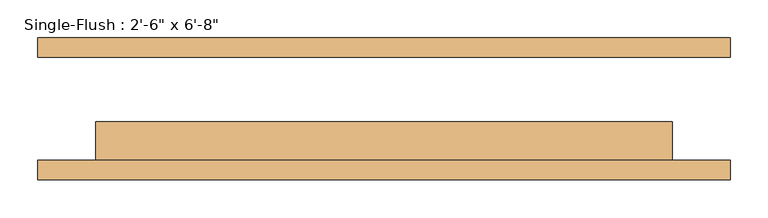
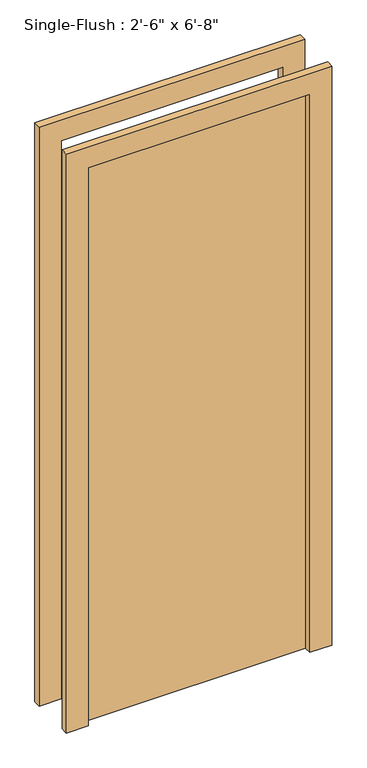
"""IFC4 building model written with IfcOpenShell, lengths in millimetres: door geometry."""

import ifcopenshell
import ifcopenshell.guid

model = None  # the IFC model being written
_history = None  # IfcOwnerHistory: only IFC2X3 demands one
_inside = {}  # id of a spatial element -> (the spatial element, [elements in it])
_under = {}  # id of a project, library or spatial element -> (it, [spatial elements below it])
_declared = {}  # id of a project -> (the project, [libraries it declares])
_typed = {}  # id of a type object -> (the type object, [elements of that type])
_made_of = {}  # id of a material, layer set ... -> (it, [elements and type objects made of it])


def new_model(schema):
    """Start an empty IFC model of exactly this schema.

    Asked for "IFC4X3", IfcOpenShell would pick the latest addendum, in which some entities
    have other attributes; the version numbers below select the first issue.
    IFC2X3 requires an IfcOwnerHistory on every rooted entity: one is made here for all.
    """
    global model, _history
    if schema == "IFC4X3":
        model = ifcopenshell.file(schema_version=(4, 3, 0, 0))
    else:
        model = ifcopenshell.file(schema=schema)
    _inside.clear()
    _under.clear()
    _declared.clear()
    _typed.clear()
    _made_of.clear()
    _history = None
    if model.schema == "IFC2X3":
        org = make("IfcOrganization", Name="unknown")
        user = make(
            "IfcPersonAndOrganization",
            ThePerson=make("IfcPerson", FamilyName="unknown"),
            TheOrganization=org,
        )
        app = make(
            "IfcApplication",
            ApplicationDeveloper=org,
            Version="unknown",
            ApplicationFullName="unknown",
            ApplicationIdentifier="unknown",
        )
        _history = make(
            "IfcOwnerHistory",
            OwningUser=user,
            OwningApplication=app,
            ChangeAction="ADDED",
            CreationDate=0,
        )
    return model


def make(cls, **values):
    """One entity of the class cls with the attributes given. An attribute that is None is left unset."""
    return model.create_entity(
        cls, **{name: value for name, value in values.items() if value is not None}
    )


def rooted(cls, **values):
    """An entity with a GlobalId (a new one), such as an element, a storey or a relation."""
    return make(cls, GlobalId=ifcopenshell.guid.new(), OwnerHistory=_history, **values)


def si_unit(unit_type, name, prefix=None):
    """IfcSIUnit, for example si_unit("LENGTHUNIT", "METRE", prefix="MILLI")."""
    return make("IfcSIUnit", UnitType=unit_type, Prefix=prefix, Name=name)


def assignment(units):
    """IfcUnitAssignment: the units of a project."""
    return None if units is None else make("IfcUnitAssignment", Units=units)


def point(xyz):
    """IfcCartesianPoint."""
    return None if xyz is None else make("IfcCartesianPoint", Coordinates=xyz)


def direction(xyz):
    """IfcDirection."""
    return None if xyz is None else make("IfcDirection", DirectionRatios=xyz)


def frame(location, z_axis=None, x_axis=None):
    """IfcAxis2Placement3D, a coordinate frame: its origin and axes. An axis left out is left unset."""
    return make(
        "IfcAxis2Placement3D",
        Location=point(location),
        Axis=direction(z_axis),
        RefDirection=direction(x_axis),
    )


def origin():
    """The frame at (0, 0, 0) with its axes left unset."""
    return frame((0.0, 0.0, 0.0))


def origin_with_axes():
    """The frame at (0, 0, 0) with the z axis (0, 0, 1) and the x axis (1, 0, 0) written out."""
    return frame((0.0, 0.0, 0.0), z_axis=(0.0, 0.0, 1.0), x_axis=(1.0, 0.0, 0.0))


def place(relative_to, where):
    """IfcLocalPlacement: puts the frame where relative to a parent placement (None: the world)."""
    return make(
        "IfcLocalPlacement", PlacementRelTo=relative_to, RelativePlacement=where
    )


def context(
    kind, dimensions, precision=None, world=None, true_north=None, identifier=None
):
    """IfcGeometricRepresentationContext, for example the 3D "Model" context."""
    return make(
        "IfcGeometricRepresentationContext",
        ContextIdentifier=identifier,
        ContextType=kind,
        CoordinateSpaceDimension=dimensions,
        Precision=precision,
        WorldCoordinateSystem=world,
        TrueNorth=true_north,
    )


def project(units=None, contexts=None):
    """IfcProject with its units and contexts."""
    return rooted(
        "IfcProject",
        Name="project",
        RepresentationContexts=contexts,
        UnitsInContext=assignment(units),
    )


def spatial(cls, under=None, at=None, **own):
    """A site, building, storey or space (cls), placed at a placement, below another one or the project."""
    s = rooted(cls, ObjectPlacement=at, **own)
    if under is not None:
        _under.setdefault(under.id(), (under, []))[1].append(s)
    return s


def polyline(points):
    """IfcPolyline through the points."""
    return make("IfcPolyline", Points=[point(p) for p in points])


def outline(outer, holes=None, kind="AREA"):
    """IfcArbitraryClosedProfileDef: a profile drawn as a closed curve; with holes, ...WithVoids."""
    if holes is None:
        return make("IfcArbitraryClosedProfileDef", ProfileType=kind, OuterCurve=outer)
    return make(
        "IfcArbitraryProfileDefWithVoids",
        ProfileType=kind,
        OuterCurve=outer,
        InnerCurves=holes,
    )


def extrude(swept, where, along, depth):
    """IfcExtrudedAreaSolid: the profile swept, set in the frame where, extruded along a direction by depth."""
    return make(
        "IfcExtrudedAreaSolid",
        SweptArea=swept,
        Position=where,
        ExtrudedDirection=direction(along),
        Depth=depth,
    )


def shape(context_of_items, identifier, shape_type, items):
    """IfcShapeRepresentation: the items that make up one representation, for example the "Body"."""
    return make(
        "IfcShapeRepresentation",
        ContextOfItems=context_of_items,
        RepresentationIdentifier=identifier,
        RepresentationType=shape_type,
        Items=items,
    )


def source(mapping_origin, context_of_items, identifier, shape_type, items):
    """IfcRepresentationMap: a shape defined once, which mapped items show again and again."""
    return make(
        "IfcRepresentationMap",
        MappingOrigin=mapping_origin,
        MappedRepresentation=shape(context_of_items, identifier, shape_type, items),
    )


def transform(
    local_origin,
    x_axis=None,
    y_axis=None,
    z_axis=None,
    scale=None,
    scale2=None,
    scale3=None,
    uniform=True,
):
    """IfcCartesianTransformationOperator3D, or its non-uniform kind. x_axis, y_axis, z_axis: its Axis1, 2, 3."""
    if uniform:
        return make(
            "IfcCartesianTransformationOperator3D",
            Axis1=direction(x_axis),
            Axis2=direction(y_axis),
            LocalOrigin=point(local_origin),
            Scale=scale,
            Axis3=direction(z_axis),
        )
    return make(
        "IfcCartesianTransformationOperator3DnonUniform",
        Axis1=direction(x_axis),
        Axis2=direction(y_axis),
        LocalOrigin=point(local_origin),
        Scale=scale,
        Axis3=direction(z_axis),
        Scale2=scale2,
        Scale3=scale3,
    )


def mapped(mapping_source, mapping_target):
    """IfcMappedItem: shows the shape of a source again, moved by a transform."""
    return make(
        "IfcMappedItem", MappingSource=mapping_source, MappingTarget=mapping_target
    )


def made_of(thing, what):
    """Note that an element or type object is made of a material, layer set ...; save() writes the relation."""
    if what is not None:
        _made_of.setdefault(what.id(), (what, []))[1].append(thing)
    return thing


def element(
    cls,
    number,
    at=None,
    inside=None,
    cuts=None,
    type_object=None,
    material=None,
    context=None,
    identifier="Body",
    shape_type=None,
    held_by="IfcProductDefinitionShape",
    body=None,
    shapes=None,
    **own,
):
    """One element of the class cls, such as IfcWall. Its Tag is "e" and its number.

    at: its placement. inside: the storey or other place that contains it. cuts: it is an
    opening in that element (IfcRelVoidsElement). A single representation is given by context,
    identifier, shape_type and body (its items); several are given by shapes. held_by: the class
    of the entity that holds the representations. save() writes the other relations.
    """
    e = rooted(cls, Tag="e%d" % number, ObjectPlacement=at, **own)
    if body is not None:
        shapes = [shape(context, identifier, shape_type, body)]
    if shapes is not None:
        e.Representation = make(held_by, Representations=shapes)
    if inside is not None:
        _inside.setdefault(inside.id(), (inside, []))[1].append(e)
    if cuts is not None:
        rooted(
            "IfcRelVoidsElement", RelatingBuildingElement=cuts, RelatedOpeningElement=e
        )
    if type_object is not None:
        _typed.setdefault(type_object.id(), (type_object, []))[1].append(e)
    return made_of(e, material)


def aggregate(whole, parts):
    """IfcRelAggregates: a whole, such as a stair, and the parts it consists of."""
    return rooted("IfcRelAggregates", RelatingObject=whole, RelatedObjects=parts)


def save(model, path):
    """Write the relations noted so far, then the file.

    IfcRelAggregates (storeys below a building ...), IfcRelContainedInSpatialStructure (elements
    in a storey), IfcRelDefinesByType, IfcRelAssociatesMaterial and IfcRelDeclares: one each for
    every whole, place, type object, material and project.
    """
    for whole, parts in _under.values():
        aggregate(whole, parts)
    for where, things in _inside.values():
        rooted(
            "IfcRelContainedInSpatialStructure",
            RelatedElements=things,
            RelatingStructure=where,
        )
    for kind, things in _typed.values():
        rooted("IfcRelDefinesByType", RelatedObjects=things, RelatingType=kind)
    for what, things in _made_of.values():
        rooted("IfcRelAssociatesMaterial", RelatedObjects=things, RelatingMaterial=what)
    for by, libraries in _declared.values():
        rooted("IfcRelDeclares", RelatingContext=by, RelatedDefinitions=libraries)
    model.write(path)


def door_cf295576(model_context):
    return source(origin(), model_context, "Body", "SweptSolid", [
        extrude(outline(polyline([(2108.2, -457.2), (0.0, -457.2), (0.0, -381.0), (2032.0, -381.0), (2032.0, 381.0), (0.0, 381.0), (0.0, 457.2), (2108.2, 457.2), (2108.2, -457.2)])), frame((0.0, -93.6625, 0.0), z_axis=(0.0, 1.0, 0.0), x_axis=(0.0, 0.0, 1.0)), (0.0, 0.0, 1.0), 25.4),
        extrude(outline(polyline([(2108.2, 457.2), (2108.2, -457.2), (0.0, -457.2), (0.0, -381.0), (2032.0, -381.0), (2032.0, 381.0), (0.0, 381.0), (0.0, 457.2), (2108.2, 457.2)])), frame((0.0, 68.2625, 0.0), z_axis=(0.0, 1.0, 0.0), x_axis=(0.0, 0.0, 1.0)), (0.0, 0.0, 1.0), 25.4),
        extrude(outline(polyline([(381.0, -17.4625), (381.0, -68.2625), (-381.0, -68.2625), (-381.0, -17.4625), (381.0, -17.4625)])), origin_with_axes(), (0.0, 0.0, 1.0), 2032.0),
    ])


if __name__ == "__main__":
    model = new_model("IFC4")
    model_context = context("Model", 3, world=origin())
    ifc_project = project(units=[si_unit("LENGTHUNIT", "METRE", prefix="MILLI")], contexts=[model_context])
    site = spatial("IfcSite", under=ifc_project)
    building = spatial("IfcBuilding", under=site)
    placement = place(None, origin())
    door_shape = door_cf295576(model_context)
    element("IfcDoor", 1, ObjectType="Single-Flush : 2'-6\" x 6'-8\"", at=placement, inside=building, context=model_context, shape_type="MappedRepresentation", body=[
        mapped(door_shape, transform((0.0, 0.0, 0.0), x_axis=(1.0, 0.0, 0.0), y_axis=(0.0, 1.0, 0.0), z_axis=(0.0, 0.0, 1.0))),
    ])
    save(model, "model.ifc")

# Revit data of these elements
# Type "Single-Flush : 2'-6\" x 6'-8\""
#   Type Mark = "13"
#   Construction Type Id = "MDOOR"
#   Assembly Code = "C1020"
#   Analytic Construction = "Metal"
#   Thickness = 0' - 2"
#   Heat Transfer Coefficient (U) = 3.7021 W/(m²·K)
#   Height = 6' - 8"
#   Trim Projection Ext = 0' - 1"
#   Trim Projection Int = 0' - 1"
#   Trim Width = 0' - 3"
#   Width = 2' - 6"
#   Door Material = Door - Panel
#   Frame Material = Door - Frame
#   Visual Light Transmittance = 0
#   Solar Heat Gain Coefficient = 0
#   Function = (empty or 0)
#   Wall Closure = (empty or 0)
# Element 1 (IfcDoor, "Single-Flush : 2'-6\" x 6'-8\"")
#   Materials on its faces: "Door - Frame", "Door - Panel"
# Materials
#   "Door - Panel": class "Wood", colour RGB 210 159 95, transparency 0, Cost = 0
#   "Door - Frame": class "Miscellaneous", colour RGB 118 70 51, transparency 0, Cost = 0
